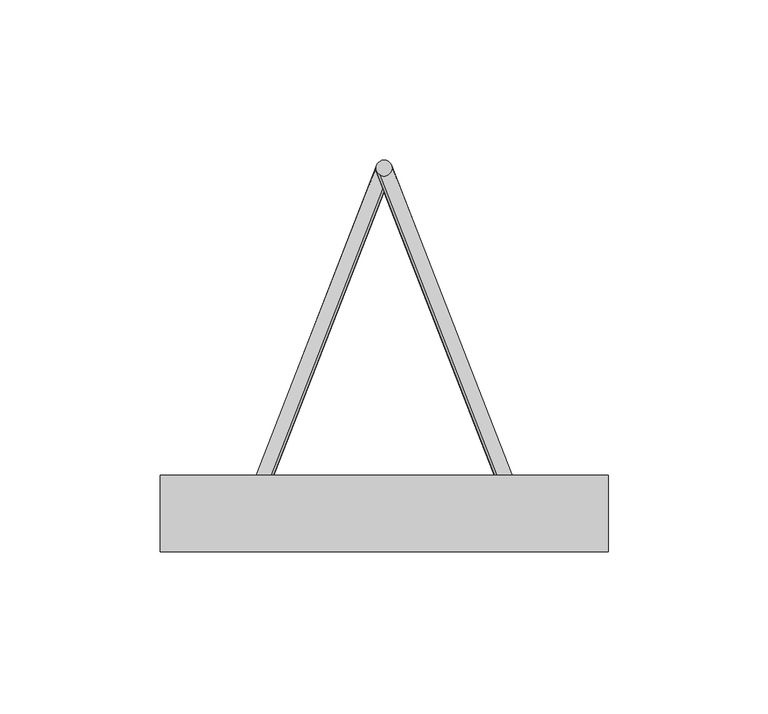
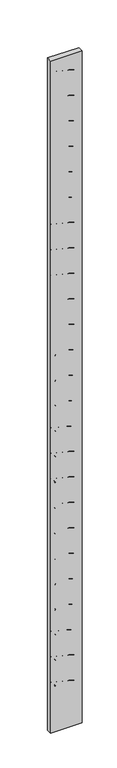
"""IFC4 building model written with IfcOpenShell, lengths in millimetres: proxy geometry, Vigota 2 (Pano 4) (Mf = 837)."""

from ifc_helpers import new_model, si_unit, point, frame, frame_2d, origin, origin_with_axes, origin_2d, place, context, project, spatial, polyline, circle_curve, trimmed, segment, composite_curve, outline, extrude, source, transform, mapped, element, save


def structural_framing_67343a58(model_context):
    return source(origin(), model_context, "Body", "SweptSolid", [
        extrude(outline(polyline([(-70.0, 12.0), (70.0, 12.0), (70.0, -12.0), (-70.0, -12.0), (-70.0, 12.0)])), origin_with_axes(), (0.0, 0.0, 1.0), 3170.0),
        extrude(outline(composite_curve([segment(trimmed(circle_curve(frame_2d((42.0, 0.0)), 2.5), [point((44.5, 0.0))], [point((39.5, 0.0))], False, "CARTESIAN"), True, "CONTINUOUS"), segment(trimmed(circle_curve(frame_2d((42.0, 0.0)), 2.5), [point((39.5, 0.0))], [point((44.5, 0.0))], False, "CARTESIAN"), True, "CONTINUOUS")], self_intersect=False)), frame((0.0, 0.0, 28.0), z_axis=(0.0, 0.0, 1.0), x_axis=(1.0, 0.0, 0.0)), (0.0, 0.0, 1.0), 3114.0),
        extrude(outline(composite_curve([segment(trimmed(circle_curve(frame_2d((0.0, 108.0)), 2.5), [point((2.5, 108.0))], [point((-2.5, 108.0))], False, "CARTESIAN"), True, "CONTINUOUS"), segment(trimmed(circle_curve(frame_2d((0.0, 108.0)), 2.5), [point((-2.5, 108.0))], [point((2.5, 108.0))], False, "CARTESIAN"), True, "CONTINUOUS")], self_intersect=False)), frame((0.0, 0.0, 95.0), z_axis=(0.0, 0.0, 1.0), x_axis=(1.0, 0.0, 0.0)), (0.0, 0.0, 1.0), 2980.0),
        extrude(outline(composite_curve([segment(trimmed(circle_curve(origin_2d(), 2.5), [point((2.5, 0.0))], [point((-2.5, 0.0))], False, "CARTESIAN"), True, "CONTINUOUS"), segment(trimmed(circle_curve(origin_2d(), 2.5), [point((-2.5, 0.0))], [point((2.5, 0.0))], False, "CARTESIAN"), True, "CONTINUOUS")], self_intersect=False)), frame((42.0, 0.0, 85.0), z_axis=(-0.3218603428886276, 0.8276408817707567, 0.4598004898837537), x_axis=(0.8192319205108605, -3.936835275445103e-11, 0.5734623443750141)), (0.0, 0.0, 1.0), 130.491379),
        extrude(outline(composite_curve([segment(trimmed(circle_curve(origin_2d(), 2.5), [point((2.5, 0.0))], [point((-2.5, 0.0))], False, "CARTESIAN"), True, "CONTINUOUS"), segment(trimmed(circle_curve(origin_2d(), 2.5), [point((-2.5, 0.0))], [point((2.5, 0.0))], False, "CARTESIAN"), True, "CONTINUOUS")], self_intersect=False)), frame((0.0, 108.0, 145.0), z_axis=(0.3218603428886276, -0.8276408817707567, 0.4598004898837537), x_axis=(0.8192319205108605, -3.936835275445103e-11, -0.5734623443750141)), (0.0, 0.0, 1.0), 130.491379),
        extrude(outline(composite_curve([segment(trimmed(circle_curve(origin_2d(), 2.5), [point((2.5, 0.0))], [point((-2.5, 0.0))], False, "CARTESIAN"), True, "CONTINUOUS"), segment(trimmed(circle_curve(origin_2d(), 2.5), [point((-2.5, 0.0))], [point((2.5, 0.0))], False, "CARTESIAN"), True, "CONTINUOUS")], self_intersect=False)), frame((42.0, 0.0, 205.0), z_axis=(-0.3218603428886276, 0.8276408817707567, 0.4598004898837537), x_axis=(0.8192319205108605, -3.936835275445103e-11, 0.5734623443750141)), (0.0, 0.0, 1.0), 130.491379),
        extrude(outline(composite_curve([segment(trimmed(circle_curve(origin_2d(), 2.5), [point((2.5, 0.0))], [point((-2.5, 0.0))], False, "CARTESIAN"), True, "CONTINUOUS"), segment(trimmed(circle_curve(origin_2d(), 2.5), [point((-2.5, 0.0))], [point((2.5, 0.0))], False, "CARTESIAN"), True, "CONTINUOUS")], self_intersect=False)), frame((0.0, 108.0, 265.0), z_axis=(0.3218603428886276, -0.8276408817707567, 0.4598004898837537), x_axis=(0.8192319205108605, -3.936835275445103e-11, -0.5734623443750141)), (0.0, 0.0, 1.0), 130.491379),
        extrude(outline(composite_curve([segment(trimmed(circle_curve(origin_2d(), 2.5), [point((2.5, 0.0))], [point((-2.5, 0.0))], False, "CARTESIAN"), True, "CONTINUOUS"), segment(trimmed(circle_curve(origin_2d(), 2.5), [point((-2.5, 0.0))], [point((2.5, 0.0))], False, "CARTESIAN"), True, "CONTINUOUS")], self_intersect=False)), frame((42.0, 0.0, 325.0), z_axis=(-0.3218603428886276, 0.8276408817707567, 0.4598004898837537), x_axis=(0.8192319205108605, -3.936835275445103e-11, 0.5734623443750141)), (0.0, 0.0, 1.0), 130.491379),
        extrude(outline(composite_curve([segment(trimmed(circle_curve(origin_2d(), 2.5), [point((2.5, 0.0))], [point((-2.5, 0.0))], False, "CARTESIAN"), True, "CONTINUOUS"), segment(trimmed(circle_curve(origin_2d(), 2.5), [point((-2.5, 0.0))], [point((2.5, 0.0))], False, "CARTESIAN"), True, "CONTINUOUS")], self_intersect=False)), frame((0.0, 108.0, 385.0), z_axis=(0.3218603428886276, -0.8276408817707567, 0.4598004898837537), x_axis=(0.8192319205108605, -3.936835275445103e-11, -0.5734623443750141)), (0.0, 0.0, 1.0), 130.491379),
        extrude(outline(composite_curve([segment(trimmed(circle_curve(origin_2d(), 2.5), [point((2.5, 0.0))], [point((-2.5, 0.0))], False, "CARTESIAN"), True, "CONTINUOUS"), segment(trimmed(circle_curve(origin_2d(), 2.5), [point((-2.5, 0.0))], [point((2.5, 0.0))], False, "CARTESIAN"), True, "CONTINUOUS")], self_intersect=False)), frame((42.0, 0.0, 445.0), z_axis=(-0.3218603428886276, 0.8276408817707567, 0.4598004898837537), x_axis=(0.8192319205108605, -3.936835275445103e-11, 0.5734623443750141)), (0.0, 0.0, 1.0), 130.491379),
        extrude(outline(composite_curve([segment(trimmed(circle_curve(origin_2d(), 2.5), [point((2.5, 0.0))], [point((-2.5, 0.0))], False, "CARTESIAN"), True, "CONTINUOUS"), segment(trimmed(circle_curve(origin_2d(), 2.5), [point((-2.5, 0.0))], [point((2.5, 0.0))], False, "CARTESIAN"), True, "CONTINUOUS")], self_intersect=False)), frame((0.0, 108.0, 505.0), z_axis=(0.3218603428886276, -0.8276408817707567, 0.4598004898837537), x_axis=(0.8192319205108605, -3.936835275445103e-11, -0.5734623443750141)), (0.0, 0.0, 1.0), 130.491379),
        extrude(outline(composite_curve([segment(trimmed(circle_curve(origin_2d(), 2.5), [point((2.5, 0.0))], [point((-2.5, 0.0))], False, "CARTESIAN"), True, "CONTINUOUS"), segment(trimmed(circle_curve(origin_2d(), 2.5), [point((-2.5, 0.0))], [point((2.5, 0.0))], False, "CARTESIAN"), True, "CONTINUOUS")], self_intersect=False)), frame((42.0, 0.0, 565.0), z_axis=(-0.3218603428886276, 0.8276408817707567, 0.4598004898837537), x_axis=(0.8192319205108605, -3.936835275445103e-11, 0.5734623443750141)), (0.0, 0.0, 1.0), 130.491379),
        extrude(outline(composite_curve([segment(trimmed(circle_curve(origin_2d(), 2.5), [point((2.5, 0.0))], [point((-2.5, 0.0))], False, "CARTESIAN"), True, "CONTINUOUS"), segment(trimmed(circle_curve(origin_2d(), 2.5), [point((-2.5, 0.0))], [point((2.5, 0.0))], False, "CARTESIAN"), True, "CONTINUOUS")], self_intersect=False)), frame((0.0, 108.0, 625.0), z_axis=(0.3218603428886276, -0.8276408817707567, 0.4598004898837537), x_axis=(0.8192319205108605, -3.936835275445103e-11, -0.5734623443750141)), (0.0, 0.0, 1.0), 130.491379),
        extrude(outline(composite_curve([segment(trimmed(circle_curve(origin_2d(), 2.5), [point((2.5, 0.0))], [point((-2.5, 0.0))], False, "CARTESIAN"), True, "CONTINUOUS"), segment(trimmed(circle_curve(origin_2d(), 2.5), [point((-2.5, 0.0))], [point((2.5, 0.0))], False, "CARTESIAN"), True, "CONTINUOUS")], self_intersect=False)), frame((42.0, 0.0, 685.0), z_axis=(-0.3218603428886276, 0.8276408817707567, 0.4598004898837537), x_axis=(0.8192319205108605, -3.936835275445103e-11, 0.5734623443750141)), (0.0, 0.0, 1.0), 130.491379),
        extrude(outline(composite_curve([segment(trimmed(circle_curve(origin_2d(), 2.5), [point((2.5, 0.0))], [point((-2.5, 0.0))], False, "CARTESIAN"), True, "CONTINUOUS"), segment(trimmed(circle_curve(origin_2d(), 2.5), [point((-2.5, 0.0))], [point((2.5, 0.0))], False, "CARTESIAN"), True, "CONTINUOUS")], self_intersect=False)), frame((0.0, 108.0, 745.0), z_axis=(0.3218603428886276, -0.8276408817707567, 0.4598004898837537), x_axis=(0.8192319205108605, -3.936835275445103e-11, -0.5734623443750141)), (0.0, 0.0, 1.0), 130.491379),
        extrude(outline(composite_curve([segment(trimmed(circle_curve(origin_2d(), 2.5), [point((2.5, 0.0))], [point((-2.5, 0.0))], False, "CARTESIAN"), True, "CONTINUOUS"), segment(trimmed(circle_curve(origin_2d(), 2.5), [point((-2.5, 0.0))], [point((2.5, 0.0))], False, "CARTESIAN"), True, "CONTINUOUS")], self_intersect=False)), frame((42.0, 0.0, 805.0), z_axis=(-0.3218603428886276, 0.8276408817707567, 0.4598004898837537), x_axis=(0.8192319205108605, -3.936835275445103e-11, 0.5734623443750141)), (0.0, 0.0, 1.0), 130.491379),
        extrude(outline(composite_curve([segment(trimmed(circle_curve(origin_2d(), 2.5), [point((2.5, 0.0))], [point((-2.5, 0.0))], False, "CARTESIAN"), True, "CONTINUOUS"), segment(trimmed(circle_curve(origin_2d(), 2.5), [point((-2.5, 0.0))], [point((2.5, 0.0))], False, "CARTESIAN"), True, "CONTINUOUS")], self_intersect=False)), frame((0.0, 108.0, 865.0), z_axis=(0.3218603428886276, -0.8276408817707567, 0.4598004898837537), x_axis=(0.8192319205108605, -3.936835275445103e-11, -0.5734623443750141)), (0.0, 0.0, 1.0), 130.491379),
        extrude(outline(composite_curve([segment(trimmed(circle_curve(origin_2d(), 2.5), [point((2.5, 0.0))], [point((-2.5, 0.0))], False, "CARTESIAN"), True, "CONTINUOUS"), segment(trimmed(circle_curve(origin_2d(), 2.5), [point((-2.5, 0.0))], [point((2.5, 0.0))], False, "CARTESIAN"), True, "CONTINUOUS")], self_intersect=False)), frame((42.0, 0.0, 925.0), z_axis=(-0.3218603428886276, 0.8276408817707567, 0.4598004898837537), x_axis=(0.8192319205108605, -3.936835275445103e-11, 0.5734623443750141)), (0.0, 0.0, 1.0), 130.491379),
        extrude(outline(composite_curve([segment(trimmed(circle_curve(origin_2d(), 2.5), [point((2.5, 0.0))], [point((-2.5, 0.0))], False, "CARTESIAN"), True, "CONTINUOUS"), segment(trimmed(circle_curve(origin_2d(), 2.5), [point((-2.5, 0.0))], [point((2.5, 0.0))], False, "CARTESIAN"), True, "CONTINUOUS")], self_intersect=False)), frame((0.0, 108.0, 985.0), z_axis=(0.3218603428886276, -0.8276408817707567, 0.4598004898837537), x_axis=(0.8192319205108605, -3.936835275445103e-11, -0.5734623443750141)), (0.0, 0.0, 1.0), 130.491379),
        extrude(outline(composite_curve([segment(trimmed(circle_curve(origin_2d(), 2.5), [point((2.5, 0.0))], [point((-2.5, 0.0))], False, "CARTESIAN"), True, "CONTINUOUS"), segment(trimmed(circle_curve(origin_2d(), 2.5), [point((-2.5, 0.0))], [point((2.5, 0.0))], False, "CARTESIAN"), True, "CONTINUOUS")], self_intersect=False)), frame((42.0, 0.0, 1045.0), z_axis=(-0.3218603428886276, 0.8276408817707567, 0.4598004898837537), x_axis=(0.8192319205108605, -3.936835275445103e-11, 0.5734623443750141)), (0.0, 0.0, 1.0), 130.491379),
        extrude(outline(composite_curve([segment(trimmed(circle_curve(origin_2d(), 2.5), [point((2.5, 0.0))], [point((-2.5, 0.0))], False, "CARTESIAN"), True, "CONTINUOUS"), segment(trimmed(circle_curve(origin_2d(), 2.5), [point((-2.5, 0.0))], [point((2.5, 0.0))], False, "CARTESIAN"), True, "CONTINUOUS")], self_intersect=False)), frame((0.0, 108.0, 1105.0), z_axis=(0.3218603428886276, -0.8276408817707567, 0.4598004898837537), x_axis=(0.8192319205108605, -3.936835275445103e-11, -0.5734623443750141)), (0.0, 0.0, 1.0), 130.491379),
        extrude(outline(composite_curve([segment(trimmed(circle_curve(origin_2d(), 2.5), [point((2.5, 0.0))], [point((-2.5, 0.0))], False, "CARTESIAN"), True, "CONTINUOUS"), segment(trimmed(circle_curve(origin_2d(), 2.5), [point((-2.5, 0.0))], [point((2.5, 0.0))], False, "CARTESIAN"), True, "CONTINUOUS")], self_intersect=False)), frame((42.0, 0.0, 1165.0), z_axis=(-0.3218603428886276, 0.8276408817707567, 0.4598004898837537), x_axis=(0.8192319205108605, -3.936835275445103e-11, 0.5734623443750141)), (0.0, 0.0, 1.0), 130.491379),
        extrude(outline(composite_curve([segment(trimmed(circle_curve(origin_2d(), 2.5), [point((2.5, 0.0))], [point((-2.5, 0.0))], False, "CARTESIAN"), True, "CONTINUOUS"), segment(trimmed(circle_curve(origin_2d(), 2.5), [point((-2.5, 0.0))], [point((2.5, 0.0))], False, "CARTESIAN"), True, "CONTINUOUS")], self_intersect=False)), frame((0.0, 108.0, 1225.0), z_axis=(0.3218603428886276, -0.8276408817707567, 0.4598004898837537), x_axis=(0.8192319205108605, -3.936835275445103e-11, -0.5734623443750141)), (0.0, 0.0, 1.0), 130.491379),
        extrude(outline(composite_curve([segment(trimmed(circle_curve(origin_2d(), 2.5), [point((2.5, 0.0))], [point((-2.5, 0.0))], False, "CARTESIAN"), True, "CONTINUOUS"), segment(trimmed(circle_curve(origin_2d(), 2.5), [point((-2.5, 0.0))], [point((2.5, 0.0))], False, "CARTESIAN"), True, "CONTINUOUS")], self_intersect=False)), frame((42.0, 0.0, 1285.0), z_axis=(-0.3218603428886276, 0.8276408817707567, 0.4598004898837537), x_axis=(0.8192319205108605, -3.936835275445103e-11, 0.5734623443750141)), (0.0, 0.0, 1.0), 130.491379),
        extrude(outline(composite_curve([segment(trimmed(circle_curve(origin_2d(), 2.5), [point((2.5, 0.0))], [point((-2.5, 0.0))], False, "CARTESIAN"), True, "CONTINUOUS"), segment(trimmed(circle_curve(origin_2d(), 2.5), [point((-2.5, 0.0))], [point((2.5, 0.0))], False, "CARTESIAN"), True, "CONTINUOUS")], self_intersect=False)), frame((0.0, 108.0, 1345.0), z_axis=(0.3218603428886276, -0.8276408817707567, 0.4598004898837537), x_axis=(0.8192319205108605, -3.936835275445103e-11, -0.5734623443750141)), (0.0, 0.0, 1.0), 130.491379),
        extrude(outline(composite_curve([segment(trimmed(circle_curve(origin_2d(), 2.5), [point((2.5, 0.0))], [point((-2.5, 0.0))], False, "CARTESIAN"), True, "CONTINUOUS"), segment(trimmed(circle_curve(origin_2d(), 2.5), [point((-2.5, 0.0))], [point((2.5, 0.0))], False, "CARTESIAN"), True, "CONTINUOUS")], self_intersect=False)), frame((42.0, 0.0, 1405.0), z_axis=(-0.3218603428886276, 0.8276408817707567, 0.4598004898837537), x_axis=(0.8192319205108605, -3.936835275445103e-11, 0.5734623443750141)), (0.0, 0.0, 1.0), 130.491379),
        extrude(outline(composite_curve([segment(trimmed(circle_curve(origin_2d(), 2.5), [point((2.5, 0.0))], [point((-2.5, 0.0))], False, "CARTESIAN"), True, "CONTINUOUS"), segment(trimmed(circle_curve(origin_2d(), 2.5), [point((-2.5, 0.0))], [point((2.5, 0.0))], False, "CARTESIAN"), True, "CONTINUOUS")], self_intersect=False)), frame((0.0, 108.0, 1465.0), z_axis=(0.3218603428886276, -0.8276408817707567, 0.4598004898837537), x_axis=(0.8192319205108605, -3.936835275445103e-11, -0.5734623443750141)), (0.0, 0.0, 1.0), 130.491379),
        extrude(outline(composite_curve([segment(trimmed(circle_curve(origin_2d(), 2.5), [point((2.5, 0.0))], [point((-2.5, 0.0))], False, "CARTESIAN"), True, "CONTINUOUS"), segment(trimmed(circle_curve(origin_2d(), 2.5), [point((-2.5, 0.0))], [point((2.5, 0.0))], False, "CARTESIAN"), True, "CONTINUOUS")], self_intersect=False)), frame((42.0, 0.0, 1525.0), z_axis=(-0.3218603428886276, 0.8276408817707567, 0.4598004898837537), x_axis=(0.8192319205108605, -3.936835275445103e-11, 0.5734623443750141)), (0.0, 0.0, 1.0), 130.491379),
        extrude(outline(composite_curve([segment(trimmed(circle_curve(origin_2d(), 2.5), [point((2.5, 0.0))], [point((-2.5, 0.0))], False, "CARTESIAN"), True, "CONTINUOUS"), segment(trimmed(circle_curve(origin_2d(), 2.5), [point((-2.5, 0.0))], [point((2.5, 0.0))], False, "CARTESIAN"), True, "CONTINUOUS")], self_intersect=False)), frame((0.0, 108.0, 1585.0), z_axis=(0.3218603428886276, -0.8276408817707567, 0.4598004898837537), x_axis=(0.8192319205108605, -3.936835275445103e-11, -0.5734623443750141)), (0.0, 0.0, 1.0), 130.491379),
        extrude(outline(composite_curve([segment(trimmed(circle_curve(origin_2d(), 2.5), [point((2.5, 0.0))], [point((-2.5, 0.0))], False, "CARTESIAN"), True, "CONTINUOUS"), segment(trimmed(circle_curve(origin_2d(), 2.5), [point((-2.5, 0.0))], [point((2.5, 0.0))], False, "CARTESIAN"), True, "CONTINUOUS")], self_intersect=False)), frame((42.0, 0.0, 1645.0), z_axis=(-0.3218603428886276, 0.8276408817707567, 0.4598004898837537), x_axis=(0.8192319205108605, -3.936835275445103e-11, 0.5734623443750141)), (0.0, 0.0, 1.0), 130.491379),
        extrude(outline(composite_curve([segment(trimmed(circle_curve(origin_2d(), 2.5), [point((2.5, 0.0))], [point((-2.5, 0.0))], False, "CARTESIAN"), True, "CONTINUOUS"), segment(trimmed(circle_curve(origin_2d(), 2.5), [point((-2.5, 0.0))], [point((2.5, 0.0))], False, "CARTESIAN"), True, "CONTINUOUS")], self_intersect=False)), frame((0.0, 108.0, 1705.0), z_axis=(0.3218603428886276, -0.8276408817707567, 0.4598004898837537), x_axis=(0.8192319205108605, -3.936835275445103e-11, -0.5734623443750141)), (0.0, 0.0, 1.0), 130.491379),
        extrude(outline(composite_curve([segment(trimmed(circle_curve(origin_2d(), 2.5), [point((2.5, 0.0))], [point((-2.5, 0.0))], False, "CARTESIAN"), True, "CONTINUOUS"), segment(trimmed(circle_curve(origin_2d(), 2.5), [point((-2.5, 0.0))], [point((2.5, 0.0))], False, "CARTESIAN"), True, "CONTINUOUS")], self_intersect=False)), frame((42.0, 0.0, 1765.0), z_axis=(-0.3218603428886276, 0.8276408817707567, 0.4598004898837537), x_axis=(0.8192319205108605, -3.936835275445103e-11, 0.5734623443750141)), (0.0, 0.0, 1.0), 130.491379),
        extrude(outline(composite_curve([segment(trimmed(circle_curve(origin_2d(), 2.5), [point((2.5, 0.0))], [point((-2.5, 0.0))], False, "CARTESIAN"), True, "CONTINUOUS"), segment(trimmed(circle_curve(origin_2d(), 2.5), [point((-2.5, 0.0))], [point((2.5, 0.0))], False, "CARTESIAN"), True, "CONTINUOUS")], self_intersect=False)), frame((0.0, 108.0, 1825.0), z_axis=(0.3218603428886276, -0.8276408817707567, 0.4598004898837537), x_axis=(0.8192319205108605, -3.936835275445103e-11, -0.5734623443750141)), (0.0, 0.0, 1.0), 130.491379),
        extrude(outline(composite_curve([segment(trimmed(circle_curve(origin_2d(), 2.5), [point((2.5, 0.0))], [point((-2.5, 0.0))], False, "CARTESIAN"), True, "CONTINUOUS"), segment(trimmed(circle_curve(origin_2d(), 2.5), [point((-2.5, 0.0))], [point((2.5, 0.0))], False, "CARTESIAN"), True, "CONTINUOUS")], self_intersect=False)), frame((42.0, 0.0, 1885.0), z_axis=(-0.3218603428886276, 0.8276408817707567, 0.4598004898837537), x_axis=(0.8192319205108605, -3.936835275445103e-11, 0.5734623443750141)), (0.0, 0.0, 1.0), 130.491379),
        extrude(outline(composite_curve([segment(trimmed(circle_curve(origin_2d(), 2.5), [point((2.5, 0.0))], [point((-2.5, 0.0))], False, "CARTESIAN"), True, "CONTINUOUS"), segment(trimmed(circle_curve(origin_2d(), 2.5), [point((-2.5, 0.0))], [point((2.5, 0.0))], False, "CARTESIAN"), True, "CONTINUOUS")], self_intersect=False)), frame((0.0, 108.0, 1945.0), z_axis=(0.3218603428886276, -0.8276408817707567, 0.4598004898837537), x_axis=(0.8192319205108605, -3.936835275445103e-11, -0.5734623443750141)), (0.0, 0.0, 1.0), 130.491379),
        extrude(outline(composite_curve([segment(trimmed(circle_curve(origin_2d(), 2.5), [point((2.5, 0.0))], [point((-2.5, 0.0))], False, "CARTESIAN"), True, "CONTINUOUS"), segment(trimmed(circle_curve(origin_2d(), 2.5), [point((-2.5, 0.0))], [point((2.5, 0.0))], False, "CARTESIAN"), True, "CONTINUOUS")], self_intersect=False)), frame((42.0, 0.0, 2005.0), z_axis=(-0.3218603428886276, 0.8276408817707567, 0.4598004898837537), x_axis=(0.8192319205108605, -3.936835275445103e-11, 0.5734623443750141)), (0.0, 0.0, 1.0), 130.491379),
        extrude(outline(composite_curve([segment(trimmed(circle_curve(origin_2d(), 2.5), [point((2.5, 0.0))], [point((-2.5, 0.0))], False, "CARTESIAN"), True, "CONTINUOUS"), segment(trimmed(circle_curve(origin_2d(), 2.5), [point((-2.5, 0.0))], [point((2.5, 0.0))], False, "CARTESIAN"), True, "CONTINUOUS")], self_intersect=False)), frame((0.0, 108.0, 2065.0), z_axis=(0.3218603428886276, -0.8276408817707567, 0.4598004898837537), x_axis=(0.8192319205108605, -3.936835275445103e-11, -0.5734623443750141)), (0.0, 0.0, 1.0), 130.491379),
        extrude(outline(composite_curve([segment(trimmed(circle_curve(origin_2d(), 2.5), [point((2.5, 0.0))], [point((-2.5, 0.0))], False, "CARTESIAN"), True, "CONTINUOUS"), segment(trimmed(circle_curve(origin_2d(), 2.5), [point((-2.5, 0.0))], [point((2.5, 0.0))], False, "CARTESIAN"), True, "CONTINUOUS")], self_intersect=False)), frame((42.0, 0.0, 2125.0), z_axis=(-0.3218603428886276, 0.8276408817707567, 0.4598004898837537), x_axis=(0.8192319205108605, -3.936835275445103e-11, 0.5734623443750141)), (0.0, 0.0, 1.0), 130.491379),
        extrude(outline(composite_curve([segment(trimmed(circle_curve(origin_2d(), 2.5), [point((2.5, 0.0))], [point((-2.5, 0.0))], False, "CARTESIAN"), True, "CONTINUOUS"), segment(trimmed(circle_curve(origin_2d(), 2.5), [point((-2.5, 0.0))], [point((2.5, 0.0))], False, "CARTESIAN"), True, "CONTINUOUS")], self_intersect=False)), frame((0.0, 108.0, 2185.0), z_axis=(0.3218603428886276, -0.8276408817707567, 0.4598004898837537), x_axis=(0.8192319205108605, -3.936835275445103e-11, -0.5734623443750141)), (0.0, 0.0, 1.0), 130.491379),
        extrude(outline(composite_curve([segment(trimmed(circle_curve(origin_2d(), 2.5), [point((2.5, 0.0))], [point((-2.5, 0.0))], False, "CARTESIAN"), True, "CONTINUOUS"), segment(trimmed(circle_curve(origin_2d(), 2.5), [point((-2.5, 0.0))], [point((2.5, 0.0))], False, "CARTESIAN"), True, "CONTINUOUS")], self_intersect=False)), frame((42.0, 0.0, 2245.0), z_axis=(-0.3218603428886276, 0.8276408817707567, 0.4598004898837537), x_axis=(0.8192319205108605, -3.936835275445103e-11, 0.5734623443750141)), (0.0, 0.0, 1.0), 130.491379),
        extrude(outline(composite_curve([segment(trimmed(circle_curve(origin_2d(), 2.5), [point((2.5, 0.0))], [point((-2.5, 0.0))], False, "CARTESIAN"), True, "CONTINUOUS"), segment(trimmed(circle_curve(origin_2d(), 2.5), [point((-2.5, 0.0))], [point((2.5, 0.0))], False, "CARTESIAN"), True, "CONTINUOUS")], self_intersect=False)), frame((0.0, 108.0, 2305.0), z_axis=(0.3218603428886276, -0.8276408817707567, 0.4598004898837537), x_axis=(0.8192319205108605, -3.936835275445103e-11, -0.5734623443750141)), (0.0, 0.0, 1.0), 130.491379),
        extrude(outline(composite_curve([segment(trimmed(circle_curve(origin_2d(), 2.5), [point((2.5, 0.0))], [point((-2.5, 0.0))], False, "CARTESIAN"), True, "CONTINUOUS"), segment(trimmed(circle_curve(origin_2d(), 2.5), [point((-2.5, 0.0))], [point((2.5, 0.0))], False, "CARTESIAN"), True, "CONTINUOUS")], self_intersect=False)), frame((42.0, 0.0, 2365.0), z_axis=(-0.3218603428886276, 0.8276408817707567, 0.4598004898837537), x_axis=(0.8192319205108605, -3.936835275445103e-11, 0.5734623443750141)), (0.0, 0.0, 1.0), 130.491379),
        extrude(outline(composite_curve([segment(trimmed(circle_curve(origin_2d(), 2.5), [point((2.5, 0.0))], [point((-2.5, 0.0))], False, "CARTESIAN"), True, "CONTINUOUS"), segment(trimmed(circle_curve(origin_2d(), 2.5), [point((-2.5, 0.0))], [point((2.5, 0.0))], False, "CARTESIAN"), True, "CONTINUOUS")], self_intersect=False)), frame((0.0, 108.0, 2425.0), z_axis=(0.3218603428886276, -0.8276408817707567, 0.4598004898837537), x_axis=(0.8192319205108605, -3.936835275445103e-11, -0.5734623443750141)), (0.0, 0.0, 1.0), 130.491379),
        extrude(outline(composite_curve([segment(trimmed(circle_curve(origin_2d(), 2.5), [point((2.5, 0.0))], [point((-2.5, 0.0))], False, "CARTESIAN"), True, "CONTINUOUS"), segment(trimmed(circle_curve(origin_2d(), 2.5), [point((-2.5, 0.0))], [point((2.5, 0.0))], False, "CARTESIAN"), True, "CONTINUOUS")], self_intersect=False)), frame((42.0, 0.0, 2485.0), z_axis=(-0.3218603428886276, 0.8276408817707567, 0.4598004898837537), x_axis=(0.8192319205108605, -3.936835275445103e-11, 0.5734623443750141)), (0.0, 0.0, 1.0), 130.491379),
        extrude(outline(composite_curve([segment(trimmed(circle_curve(origin_2d(), 2.5), [point((2.5, 0.0))], [point((-2.5, 0.0))], False, "CARTESIAN"), True, "CONTINUOUS"), segment(trimmed(circle_curve(origin_2d(), 2.5), [point((-2.5, 0.0))], [point((2.5, 0.0))], False, "CARTESIAN"), True, "CONTINUOUS")], self_intersect=False)), frame((0.0, 108.0, 2545.0), z_axis=(0.3218603428886276, -0.8276408817707567, 0.4598004898837537), x_axis=(0.8192319205108605, -3.936835275445103e-11, -0.5734623443750141)), (0.0, 0.0, 1.0), 130.491379),
        extrude(outline(composite_curve([segment(trimmed(circle_curve(origin_2d(), 2.5), [point((2.5, 0.0))], [point((-2.5, 0.0))], False, "CARTESIAN"), True, "CONTINUOUS"), segment(trimmed(circle_curve(origin_2d(), 2.5), [point((-2.5, 0.0))], [point((2.5, 0.0))], False, "CARTESIAN"), True, "CONTINUOUS")], self_intersect=False)), frame((42.0, 0.0, 2605.0), z_axis=(-0.3218603428886276, 0.8276408817707567, 0.4598004898837537), x_axis=(0.8192319205108605, -3.936835275445103e-11, 0.5734623443750141)), (0.0, 0.0, 1.0), 130.491379),
        extrude(outline(composite_curve([segment(trimmed(circle_curve(origin_2d(), 2.5), [point((2.5, 0.0))], [point((-2.5, 0.0))], False, "CARTESIAN"), True, "CONTINUOUS"), segment(trimmed(circle_curve(origin_2d(), 2.5), [point((-2.5, 0.0))], [point((2.5, 0.0))], False, "CARTESIAN"), True, "CONTINUOUS")], self_intersect=False)), frame((0.0, 108.0, 2665.0), z_axis=(0.3218603428886276, -0.8276408817707567, 0.4598004898837537), x_axis=(0.8192319205108605, -3.936835275445103e-11, -0.5734623443750141)), (0.0, 0.0, 1.0), 130.491379),
        extrude(outline(composite_curve([segment(trimmed(circle_curve(origin_2d(), 2.5), [point((2.5, 0.0))], [point((-2.5, 0.0))], False, "CARTESIAN"), True, "CONTINUOUS"), segment(trimmed(circle_curve(origin_2d(), 2.5), [point((-2.5, 0.0))], [point((2.5, 0.0))], False, "CARTESIAN"), True, "CONTINUOUS")], self_intersect=False)), frame((42.0, 0.0, 2725.0), z_axis=(-0.3218603428886276, 0.8276408817707567, 0.4598004898837537), x_axis=(0.8192319205108605, -3.936835275445103e-11, 0.5734623443750141)), (0.0, 0.0, 1.0), 130.491379),
        extrude(outline(composite_curve([segment(trimmed(circle_curve(origin_2d(), 2.5), [point((2.5, 0.0))], [point((-2.5, 0.0))], False, "CARTESIAN"), True, "CONTINUOUS"), segment(trimmed(circle_curve(origin_2d(), 2.5), [point((-2.5, 0.0))], [point((2.5, 0.0))], False, "CARTESIAN"), True, "CONTINUOUS")], self_intersect=False)), frame((0.0, 108.0, 2785.0), z_axis=(0.3218603428886276, -0.8276408817707567, 0.4598004898837537), x_axis=(0.8192319205108605, -3.936835275445103e-11, -0.5734623443750141)), (0.0, 0.0, 1.0), 130.491379),
        extrude(outline(composite_curve([segment(trimmed(circle_curve(origin_2d(), 2.5), [point((2.5, 0.0))], [point((-2.5, 0.0))], False, "CARTESIAN"), True, "CONTINUOUS"), segment(trimmed(circle_curve(origin_2d(), 2.5), [point((-2.5, 0.0))], [point((2.5, 0.0))], False, "CARTESIAN"), True, "CONTINUOUS")], self_intersect=False)), frame((42.0, 0.0, 2845.0), z_axis=(-0.3218603428886276, 0.8276408817707567, 0.4598004898837537), x_axis=(0.8192319205108605, -3.936835275445103e-11, 0.5734623443750141)), (0.0, 0.0, 1.0), 130.491379),
        extrude(outline(composite_curve([segment(trimmed(circle_curve(origin_2d(), 2.5), [point((2.5, 0.0))], [point((-2.5, 0.0))], False, "CARTESIAN"), True, "CONTINUOUS"), segment(trimmed(circle_curve(origin_2d(), 2.5), [point((-2.5, 0.0))], [point((2.5, 0.0))], False, "CARTESIAN"), True, "CONTINUOUS")], self_intersect=False)), frame((0.0, 108.0, 2905.0), z_axis=(0.3218603428886276, -0.8276408817707567, 0.4598004898837537), x_axis=(0.8192319205108605, -3.936835275445103e-11, -0.5734623443750141)), (0.0, 0.0, 1.0), 130.491379),
        extrude(outline(composite_curve([segment(trimmed(circle_curve(origin_2d(), 2.5), [point((2.5, 0.0))], [point((-2.5, 0.0))], False, "CARTESIAN"), True, "CONTINUOUS"), segment(trimmed(circle_curve(origin_2d(), 2.5), [point((-2.5, 0.0))], [point((2.5, 0.0))], False, "CARTESIAN"), True, "CONTINUOUS")], self_intersect=False)), frame((42.0, 0.0, 2965.0), z_axis=(-0.3218603428886276, 0.8276408817707567, 0.4598004898837537), x_axis=(0.8192319205108605, -3.936835275445103e-11, 0.5734623443750141)), (0.0, 0.0, 1.0), 130.491379),
        extrude(outline(composite_curve([segment(trimmed(circle_curve(origin_2d(), 2.5), [point((2.5, 0.0))], [point((-2.5, 0.0))], False, "CARTESIAN"), True, "CONTINUOUS"), segment(trimmed(circle_curve(origin_2d(), 2.5), [point((-2.5, 0.0))], [point((2.5, 0.0))], False, "CARTESIAN"), True, "CONTINUOUS")], self_intersect=False)), frame((0.0, 108.0, 3025.0), z_axis=(0.3218603428886276, -0.8276408817707567, 0.4598004898837537), x_axis=(0.8192319205108605, -3.936835275445103e-11, -0.5734623443750141)), (0.0, 0.0, 1.0), 130.491379),
        extrude(outline(composite_curve([segment(trimmed(circle_curve(frame_2d((-42.0, 0.0)), 2.5), [point((-39.5, 0.0))], [point((-44.5, 0.0))], False, "CARTESIAN"), True, "CONTINUOUS"), segment(trimmed(circle_curve(frame_2d((-42.0, 0.0)), 2.5), [point((-44.5, 0.0))], [point((-39.5, 0.0))], False, "CARTESIAN"), True, "CONTINUOUS")], self_intersect=False)), frame((0.0, 0.0, 28.0), z_axis=(0.0, 0.0, 1.0), x_axis=(1.0, 0.0, 0.0)), (0.0, 0.0, 1.0), 3114.0),
        extrude(outline(composite_curve([segment(trimmed(circle_curve(origin_2d(), 2.5), [point((2.5, 0.0))], [point((-2.5, 0.0))], False, "CARTESIAN"), True, "CONTINUOUS"), segment(trimmed(circle_curve(origin_2d(), 2.5), [point((-2.5, 0.0))], [point((2.5, 0.0))], False, "CARTESIAN"), True, "CONTINUOUS")], self_intersect=False)), frame((-42.0, 0.0, 85.0), z_axis=(0.3218603428886276, 0.8276408817707567, 0.4598004898837537), x_axis=(0.8192319205108605, 3.936835275445103e-11, -0.5734623443750141)), (0.0, 0.0, 1.0), 130.491379),
        extrude(outline(composite_curve([segment(trimmed(circle_curve(origin_2d(), 2.5), [point((2.5, 0.0))], [point((-2.5, 0.0))], False, "CARTESIAN"), True, "CONTINUOUS"), segment(trimmed(circle_curve(origin_2d(), 2.5), [point((-2.5, 0.0))], [point((2.5, 0.0))], False, "CARTESIAN"), True, "CONTINUOUS")], self_intersect=False)), frame((0.0, 108.0, 145.0), z_axis=(-0.3218603428886276, -0.8276408817707567, 0.4598004898837537), x_axis=(0.8192319205108605, 3.936835275445103e-11, 0.5734623443750141)), (0.0, 0.0, 1.0), 130.491379),
        extrude(outline(composite_curve([segment(trimmed(circle_curve(origin_2d(), 2.5), [point((2.5, 0.0))], [point((-2.5, 0.0))], False, "CARTESIAN"), True, "CONTINUOUS"), segment(trimmed(circle_curve(origin_2d(), 2.5), [point((-2.5, 0.0))], [point((2.5, 0.0))], False, "CARTESIAN"), True, "CONTINUOUS")], self_intersect=False)), frame((-42.0, 0.0, 205.0), z_axis=(0.3218603428886276, 0.8276408817707567, 0.4598004898837537), x_axis=(0.8192319205108605, 3.936835275445103e-11, -0.5734623443750141)), (0.0, 0.0, 1.0), 130.491379),
        extrude(outline(composite_curve([segment(trimmed(circle_curve(origin_2d(), 2.5), [point((2.5, 0.0))], [point((-2.5, 0.0))], False, "CARTESIAN"), True, "CONTINUOUS"), segment(trimmed(circle_curve(origin_2d(), 2.5), [point((-2.5, 0.0))], [point((2.5, 0.0))], False, "CARTESIAN"), True, "CONTINUOUS")], self_intersect=False)), frame((0.0, 108.0, 265.0), z_axis=(-0.3218603428886276, -0.8276408817707567, 0.4598004898837537), x_axis=(0.8192319205108605, 3.936835275445103e-11, 0.5734623443750141)), (0.0, 0.0, 1.0), 130.491379),
        extrude(outline(composite_curve([segment(trimmed(circle_curve(origin_2d(), 2.5), [point((2.5, 0.0))], [point((-2.5, 0.0))], False, "CARTESIAN"), True, "CONTINUOUS"), segment(trimmed(circle_curve(origin_2d(), 2.5), [point((-2.5, 0.0))], [point((2.5, 0.0))], False, "CARTESIAN"), True, "CONTINUOUS")], self_intersect=False)), frame((-42.0, 0.0, 325.0), z_axis=(0.3218603428886276, 0.8276408817707567, 0.4598004898837537), x_axis=(0.8192319205108605, 3.936835275445103e-11, -0.5734623443750141)), (0.0, 0.0, 1.0), 130.491379),
        extrude(outline(composite_curve([segment(trimmed(circle_curve(origin_2d(), 2.5), [point((2.5, 0.0))], [point((-2.5, 0.0))], False, "CARTESIAN"), True, "CONTINUOUS"), segment(trimmed(circle_curve(origin_2d(), 2.5), [point((-2.5, 0.0))], [point((2.5, 0.0))], False, "CARTESIAN"), True, "CONTINUOUS")], self_intersect=False)), frame((0.0, 108.0, 385.0), z_axis=(-0.3218603428886276, -0.8276408817707567, 0.4598004898837537), x_axis=(0.8192319205108605, 3.936835275445103e-11, 0.5734623443750141)), (0.0, 0.0, 1.0), 130.491379),
        extrude(outline(composite_curve([segment(trimmed(circle_curve(origin_2d(), 2.5), [point((2.5, 0.0))], [point((-2.5, 0.0))], False, "CARTESIAN"), True, "CONTINUOUS"), segment(trimmed(circle_curve(origin_2d(), 2.5), [point((-2.5, 0.0))], [point((2.5, 0.0))], False, "CARTESIAN"), True, "CONTINUOUS")], self_intersect=False)), frame((-42.0, 0.0, 445.0), z_axis=(0.3218603428886276, 0.8276408817707567, 0.4598004898837537), x_axis=(0.8192319205108605, 3.936835275445103e-11, -0.5734623443750141)), (0.0, 0.0, 1.0), 130.491379),
        extrude(outline(composite_curve([segment(trimmed(circle_curve(origin_2d(), 2.5), [point((2.5, 0.0))], [point((-2.5, 0.0))], False, "CARTESIAN"), True, "CONTINUOUS"), segment(trimmed(circle_curve(origin_2d(), 2.5), [point((-2.5, 0.0))], [point((2.5, 0.0))], False, "CARTESIAN"), True, "CONTINUOUS")], self_intersect=False)), frame((0.0, 108.0, 505.0), z_axis=(-0.3218603428886276, -0.8276408817707567, 0.4598004898837537), x_axis=(0.8192319205108605, 3.936835275445103e-11, 0.5734623443750141)), (0.0, 0.0, 1.0), 130.491379),
        extrude(outline(composite_curve([segment(trimmed(circle_curve(origin_2d(), 2.5), [point((2.5, 0.0))], [point((-2.5, 0.0))], False, "CARTESIAN"), True, "CONTINUOUS"), segment(trimmed(circle_curve(origin_2d(), 2.5), [point((-2.5, 0.0))], [point((2.5, 0.0))], False, "CARTESIAN"), True, "CONTINUOUS")], self_intersect=False)), frame((-42.0, 0.0, 565.0), z_axis=(0.3218603428886276, 0.8276408817707567, 0.4598004898837537), x_axis=(0.8192319205108605, 3.936835275445103e-11, -0.5734623443750141)), (0.0, 0.0, 1.0), 130.491379),
        extrude(outline(composite_curve([segment(trimmed(circle_curve(origin_2d(), 2.5), [point((2.5, 0.0))], [point((-2.5, 0.0))], False, "CARTESIAN"), True, "CONTINUOUS"), segment(trimmed(circle_curve(origin_2d(), 2.5), [point((-2.5, 0.0))], [point((2.5, 0.0))], False, "CARTESIAN"), True, "CONTINUOUS")], self_intersect=False)), frame((0.0, 108.0, 625.0), z_axis=(-0.3218603428886276, -0.8276408817707567, 0.4598004898837537), x_axis=(0.8192319205108605, 3.936835275445103e-11, 0.5734623443750141)), (0.0, 0.0, 1.0), 130.491379),
        extrude(outline(composite_curve([segment(trimmed(circle_curve(origin_2d(), 2.5), [point((2.5, 0.0))], [point((-2.5, 0.0))], False, "CARTESIAN"), True, "CONTINUOUS"), segment(trimmed(circle_curve(origin_2d(), 2.5), [point((-2.5, 0.0))], [point((2.5, 0.0))], False, "CARTESIAN"), True, "CONTINUOUS")], self_intersect=False)), frame((-42.0, 0.0, 685.0), z_axis=(0.3218603428886276, 0.8276408817707567, 0.4598004898837537), x_axis=(0.8192319205108605, 3.936835275445103e-11, -0.5734623443750141)), (0.0, 0.0, 1.0), 130.491379),
        extrude(outline(composite_curve([segment(trimmed(circle_curve(origin_2d(), 2.5), [point((2.5, 0.0))], [point((-2.5, 0.0))], False, "CARTESIAN"), True, "CONTINUOUS"), segment(trimmed(circle_curve(origin_2d(), 2.5), [point((-2.5, 0.0))], [point((2.5, 0.0))], False, "CARTESIAN"), True, "CONTINUOUS")], self_intersect=False)), frame((0.0, 108.0, 745.0), z_axis=(-0.3218603428886276, -0.8276408817707567, 0.4598004898837537), x_axis=(0.8192319205108605, 3.936835275445103e-11, 0.5734623443750141)), (0.0, 0.0, 1.0), 130.491379),
        extrude(outline(composite_curve([segment(trimmed(circle_curve(origin_2d(), 2.5), [point((2.5, 0.0))], [point((-2.5, 0.0))], False, "CARTESIAN"), True, "CONTINUOUS"), segment(trimmed(circle_curve(origin_2d(), 2.5), [point((-2.5, 0.0))], [point((2.5, 0.0))], False, "CARTESIAN"), True, "CONTINUOUS")], self_intersect=False)), frame((-42.0, 0.0, 805.0), z_axis=(0.3218603428886276, 0.8276408817707567, 0.4598004898837537), x_axis=(0.8192319205108605, 3.936835275445103e-11, -0.5734623443750141)), (0.0, 0.0, 1.0), 130.491379),
        extrude(outline(composite_curve([segment(trimmed(circle_curve(origin_2d(), 2.5), [point((2.5, 0.0))], [point((-2.5, 0.0))], False, "CARTESIAN"), True, "CONTINUOUS"), segment(trimmed(circle_curve(origin_2d(), 2.5), [point((-2.5, 0.0))], [point((2.5, 0.0))], False, "CARTESIAN"), True, "CONTINUOUS")], self_intersect=False)), frame((0.0, 108.0, 865.0), z_axis=(-0.3218603428886276, -0.8276408817707567, 0.4598004898837537), x_axis=(0.8192319205108605, 3.936835275445103e-11, 0.5734623443750141)), (0.0, 0.0, 1.0), 130.491379),
        extrude(outline(composite_curve([segment(trimmed(circle_curve(origin_2d(), 2.5), [point((2.5, 0.0))], [point((-2.5, 0.0))], False, "CARTESIAN"), True, "CONTINUOUS"), segment(trimmed(circle_curve(origin_2d(), 2.5), [point((-2.5, 0.0))], [point((2.5, 0.0))], False, "CARTESIAN"), True, "CONTINUOUS")], self_intersect=False)), frame((-42.0, 0.0, 925.0), z_axis=(0.3218603428886276, 0.8276408817707567, 0.4598004898837537), x_axis=(0.8192319205108605, 3.936835275445103e-11, -0.5734623443750141)), (0.0, 0.0, 1.0), 130.491379),
        extrude(outline(composite_curve([segment(trimmed(circle_curve(origin_2d(), 2.5), [point((2.5, 0.0))], [point((-2.5, 0.0))], False, "CARTESIAN"), True, "CONTINUOUS"), segment(trimmed(circle_curve(origin_2d(), 2.5), [point((-2.5, 0.0))], [point((2.5, 0.0))], False, "CARTESIAN"), True, "CONTINUOUS")], self_intersect=False)), frame((0.0, 108.0, 985.0), z_axis=(-0.3218603428886276, -0.8276408817707567, 0.4598004898837537), x_axis=(0.8192319205108605, 3.936835275445103e-11, 0.5734623443750141)), (0.0, 0.0, 1.0), 130.491379),
        extrude(outline(composite_curve([segment(trimmed(circle_curve(origin_2d(), 2.5), [point((2.5, 0.0))], [point((-2.5, 0.0))], False, "CARTESIAN"), True, "CONTINUOUS"), segment(trimmed(circle_curve(origin_2d(), 2.5), [point((-2.5, 0.0))], [point((2.5, 0.0))], False, "CARTESIAN"), True, "CONTINUOUS")], self_intersect=False)), frame((-42.0, 0.0, 1045.0), z_axis=(0.3218603428886276, 0.8276408817707567, 0.4598004898837537), x_axis=(0.8192319205108605, 3.936835275445103e-11, -0.5734623443750141)), (0.0, 0.0, 1.0), 130.491379),
        extrude(outline(composite_curve([segment(trimmed(circle_curve(origin_2d(), 2.5), [point((2.5, 0.0))], [point((-2.5, 0.0))], False, "CARTESIAN"), True, "CONTINUOUS"), segment(trimmed(circle_curve(origin_2d(), 2.5), [point((-2.5, 0.0))], [point((2.5, 0.0))], False, "CARTESIAN"), True, "CONTINUOUS")], self_intersect=False)), frame((0.0, 108.0, 1105.0), z_axis=(-0.3218603428886276, -0.8276408817707567, 0.4598004898837537), x_axis=(0.8192319205108605, 3.936835275445103e-11, 0.5734623443750141)), (0.0, 0.0, 1.0), 130.491379),
        extrude(outline(composite_curve([segment(trimmed(circle_curve(origin_2d(), 2.5), [point((2.5, 0.0))], [point((-2.5, 0.0))], False, "CARTESIAN"), True, "CONTINUOUS"), segment(trimmed(circle_curve(origin_2d(), 2.5), [point((-2.5, 0.0))], [point((2.5, 0.0))], False, "CARTESIAN"), True, "CONTINUOUS")], self_intersect=False)), frame((-42.0, 0.0, 1165.0), z_axis=(0.3218603428886276, 0.8276408817707567, 0.4598004898837537), x_axis=(0.8192319205108605, 3.936835275445103e-11, -0.5734623443750141)), (0.0, 0.0, 1.0), 130.491379),
        extrude(outline(composite_curve([segment(trimmed(circle_curve(origin_2d(), 2.5), [point((2.5, 0.0))], [point((-2.5, 0.0))], False, "CARTESIAN"), True, "CONTINUOUS"), segment(trimmed(circle_curve(origin_2d(), 2.5), [point((-2.5, 0.0))], [point((2.5, 0.0))], False, "CARTESIAN"), True, "CONTINUOUS")], self_intersect=False)), frame((0.0, 108.0, 1225.0), z_axis=(-0.3218603428886276, -0.8276408817707567, 0.4598004898837537), x_axis=(0.8192319205108605, 3.936835275445103e-11, 0.5734623443750141)), (0.0, 0.0, 1.0), 130.491379),
        extrude(outline(composite_curve([segment(trimmed(circle_curve(origin_2d(), 2.5), [point((2.5, 0.0))], [point((-2.5, 0.0))], False, "CARTESIAN"), True, "CONTINUOUS"), segment(trimmed(circle_curve(origin_2d(), 2.5), [point((-2.5, 0.0))], [point((2.5, 0.0))], False, "CARTESIAN"), True, "CONTINUOUS")], self_intersect=False)), frame((-42.0, 0.0, 1285.0), z_axis=(0.3218603428886276, 0.8276408817707567, 0.4598004898837537), x_axis=(0.8192319205108605, 3.936835275445103e-11, -0.5734623443750141)), (0.0, 0.0, 1.0), 130.491379),
        extrude(outline(composite_curve([segment(trimmed(circle_curve(origin_2d(), 2.5), [point((2.5, 0.0))], [point((-2.5, 0.0))], False, "CARTESIAN"), True, "CONTINUOUS"), segment(trimmed(circle_curve(origin_2d(), 2.5), [point((-2.5, 0.0))], [point((2.5, 0.0))], False, "CARTESIAN"), True, "CONTINUOUS")], self_intersect=False)), frame((0.0, 108.0, 1345.0), z_axis=(-0.3218603428886276, -0.8276408817707567, 0.4598004898837537), x_axis=(0.8192319205108605, 3.936835275445103e-11, 0.5734623443750141)), (0.0, 0.0, 1.0), 130.491379),
        extrude(outline(composite_curve([segment(trimmed(circle_curve(origin_2d(), 2.5), [point((2.5, 0.0))], [point((-2.5, 0.0))], False, "CARTESIAN"), True, "CONTINUOUS"), segment(trimmed(circle_curve(origin_2d(), 2.5), [point((-2.5, 0.0))], [point((2.5, 0.0))], False, "CARTESIAN"), True, "CONTINUOUS")], self_intersect=False)), frame((-42.0, 0.0, 1405.0), z_axis=(0.3218603428886276, 0.8276408817707567, 0.4598004898837537), x_axis=(0.8192319205108605, 3.936835275445103e-11, -0.5734623443750141)), (0.0, 0.0, 1.0), 130.491379),
        extrude(outline(composite_curve([segment(trimmed(circle_curve(origin_2d(), 2.5), [point((2.5, 0.0))], [point((-2.5, 0.0))], False, "CARTESIAN"), True, "CONTINUOUS"), segment(trimmed(circle_curve(origin_2d(), 2.5), [point((-2.5, 0.0))], [point((2.5, 0.0))], False, "CARTESIAN"), True, "CONTINUOUS")], self_intersect=False)), frame((0.0, 108.0, 1465.0), z_axis=(-0.3218603428886276, -0.8276408817707567, 0.4598004898837537), x_axis=(0.8192319205108605, 3.936835275445103e-11, 0.5734623443750141)), (0.0, 0.0, 1.0), 130.491379),
        extrude(outline(composite_curve([segment(trimmed(circle_curve(origin_2d(), 2.5), [point((2.5, 0.0))], [point((-2.5, 0.0))], False, "CARTESIAN"), True, "CONTINUOUS"), segment(trimmed(circle_curve(origin_2d(), 2.5), [point((-2.5, 0.0))], [point((2.5, 0.0))], False, "CARTESIAN"), True, "CONTINUOUS")], self_intersect=False)), frame((-42.0, 0.0, 1525.0), z_axis=(0.3218603428886276, 0.8276408817707567, 0.4598004898837537), x_axis=(0.8192319205108605, 3.936835275445103e-11, -0.5734623443750141)), (0.0, 0.0, 1.0), 130.491379),
        extrude(outline(composite_curve([segment(trimmed(circle_curve(origin_2d(), 2.5), [point((2.5, 0.0))], [point((-2.5, 0.0))], False, "CARTESIAN"), True, "CONTINUOUS"), segment(trimmed(circle_curve(origin_2d(), 2.5), [point((-2.5, 0.0))], [point((2.5, 0.0))], False, "CARTESIAN"), True, "CONTINUOUS")], self_intersect=False)), frame((0.0, 108.0, 1585.0), z_axis=(-0.3218603428886276, -0.8276408817707567, 0.4598004898837537), x_axis=(0.8192319205108605, 3.936835275445103e-11, 0.5734623443750141)), (0.0, 0.0, 1.0), 130.491379),
        extrude(outline(composite_curve([segment(trimmed(circle_curve(origin_2d(), 2.5), [point((2.5, 0.0))], [point((-2.5, 0.0))], False, "CARTESIAN"), True, "CONTINUOUS"), segment(trimmed(circle_curve(origin_2d(), 2.5), [point((-2.5, 0.0))], [point((2.5, 0.0))], False, "CARTESIAN"), True, "CONTINUOUS")], self_intersect=False)), frame((-42.0, 0.0, 1645.0), z_axis=(0.3218603428886276, 0.8276408817707567, 0.4598004898837537), x_axis=(0.8192319205108605, 3.936835275445103e-11, -0.5734623443750141)), (0.0, 0.0, 1.0), 130.491379),
        extrude(outline(composite_curve([segment(trimmed(circle_curve(origin_2d(), 2.5), [point((2.5, 0.0))], [point((-2.5, 0.0))], False, "CARTESIAN"), True, "CONTINUOUS"), segment(trimmed(circle_curve(origin_2d(), 2.5), [point((-2.5, 0.0))], [point((2.5, 0.0))], False, "CARTESIAN"), True, "CONTINUOUS")], self_intersect=False)), frame((0.0, 108.0, 1705.0), z_axis=(-0.3218603428886276, -0.8276408817707567, 0.4598004898837537), x_axis=(0.8192319205108605, 3.936835275445103e-11, 0.5734623443750141)), (0.0, 0.0, 1.0), 130.491379),
    ])


if __name__ == "__main__":
    model = new_model("IFC4")
    model_context = context("Model", 3, world=origin())
    ifc_project = project(units=[si_unit("LENGTHUNIT", "METRE", prefix="MILLI")], contexts=[model_context])
    site = spatial("IfcSite", under=ifc_project)
    building = spatial("IfcBuilding", under=site)
    placement = place(None, origin())
    structural_framing_shape = structural_framing_67343a58(model_context)
    element("IfcBuildingElementProxy", 1, Name="Vigota 2 (Pano 4) (Mf = 837)", ObjectType="Vigota 2 (Pano 4) (Mf = 837)", at=placement, inside=building, context=model_context, shape_type="MappedRepresentation", body=[
        mapped(structural_framing_shape, transform((0.0, 0.0, 0.0), x_axis=(1.0, 0.0, 0.0), y_axis=(0.0, 1.0, 0.0), z_axis=(0.0, 0.0, 1.0))),
    ])
    save(model, "model.ifc")

# Revit data of these elements
# Element 1 (IfcBuildingElementProxy, "Vigota 2 (Pano 4) (Mf = 837)")
#   Materials on its faces: "Aço", "Concreto armado"
# Materials
#   "Aço": class "Metal", colour RGB 120 120 120, transparency 0, Description = "Aço estrutural A36 grau, ASTM B, acabamento laminado", Cost = 0
#   "Concreto armado": class "Não atribuído", colour RGB 168 169 158, transparency 0
